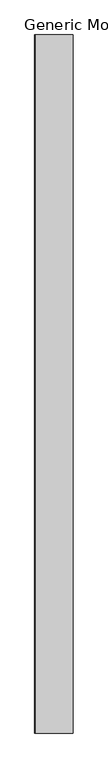
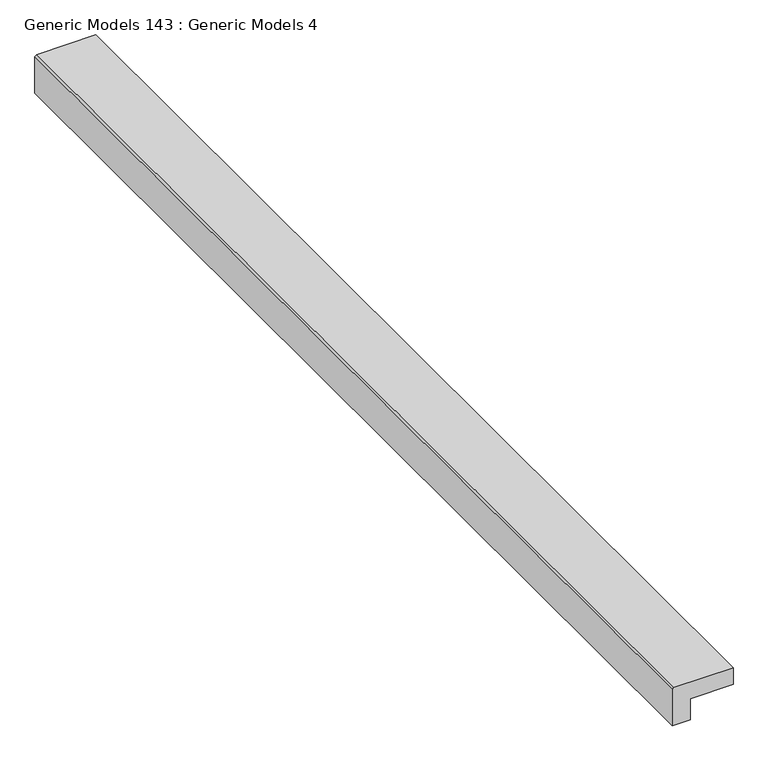
"""IFC4 building model written with IfcOpenShell, lengths in millimetres: proxy geometry, Generic Models 143 : Generic Models 4."""

from ifc_helpers import new_model, si_unit, frame, origin, place, context, project, spatial, polyline, outline, extrude, source, transform, mapped, element, save


def generic_models_143_generic_models_4_03561a33(model_context):
    return source(origin(), model_context, "Body", "SweptSolid", [
        extrude(outline(polyline([(123240.546, -6629.5736296), (122802.396, -6629.5736296), (122802.396, -6426.3736296), (123056.396, -6426.3736296), (123056.396, -5937.4236296), (123259.596, -5937.4236296), (123259.596, -6610.5236296), (123240.546, -6629.5736296)])), frame((0.0, -5493.3230338, 0.0), z_axis=(0.0, 1.0, 0.0), x_axis=(0.0, 0.0, 1.0)), (0.0, 0.0, 1.0), 12547.6),
    ])


if __name__ == "__main__":
    model = new_model("IFC4")
    model_context = context("Model", 3, world=origin())
    ifc_project = project(units=[si_unit("LENGTHUNIT", "METRE", prefix="MILLI")], contexts=[model_context])
    site = spatial("IfcSite", under=ifc_project)
    building = spatial("IfcBuilding", under=site)
    placement = place(None, origin())
    generic_models_143_generic_models_4_shape = generic_models_143_generic_models_4_03561a33(model_context)
    element("IfcBuildingElementProxy", 1, Name="Generic Models 143 : Generic Models 4", ObjectType="Generic Models 143 : Generic Models 4", at=placement, inside=building, context=model_context, shape_type="MappedRepresentation", body=[
        mapped(generic_models_143_generic_models_4_shape, transform((0.0, 0.0, 0.0), x_axis=(1.0, 0.0, 0.0), y_axis=(0.0, 1.0, 0.0), z_axis=(0.0, 0.0, 1.0))),
    ])
    save(model, "model.ifc")

# Revit data of these elements
# Element 1 (IfcBuildingElementProxy, "Generic Models 143 : Generic Models 4")
#   Materials on its faces: "_ 8\" CONCRETE SLAB W/ GRADE BEAM (SEE STRUCT. DWGS)"
# Materials
#   "_ 8\" CONCRETE SLAB W/ GRADE BEAM (SEE STRUCT. DWGS)": class "Generic", colour RGB 191 191 191, transparency 0, Cost = 0
